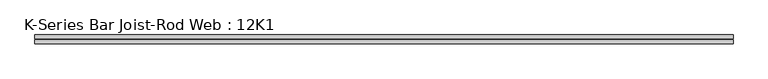
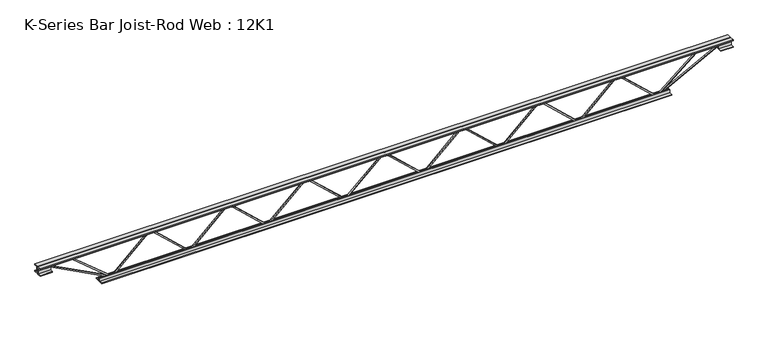
"""IFC4 building model written with IfcOpenShell, lengths in millimetres: beam geometry, K-Series Bar Joist-Rod Web : 12K1."""

import ifcopenshell
import ifcopenshell.guid

model = None  # the IFC model being written
_history = None  # IfcOwnerHistory: only IFC2X3 demands one
_inside = {}  # id of a spatial element -> (the spatial element, [elements in it])
_under = {}  # id of a project, library or spatial element -> (it, [spatial elements below it])
_declared = {}  # id of a project -> (the project, [libraries it declares])
_typed = {}  # id of a type object -> (the type object, [elements of that type])
_made_of = {}  # id of a material, layer set ... -> (it, [elements and type objects made of it])


def new_model(schema):
    """Start an empty IFC model of exactly this schema.

    Asked for "IFC4X3", IfcOpenShell would pick the latest addendum, in which some entities
    have other attributes; the version numbers below select the first issue.
    IFC2X3 requires an IfcOwnerHistory on every rooted entity: one is made here for all.
    """
    global model, _history
    if schema == "IFC4X3":
        model = ifcopenshell.file(schema_version=(4, 3, 0, 0))
    else:
        model = ifcopenshell.file(schema=schema)
    _inside.clear()
    _under.clear()
    _declared.clear()
    _typed.clear()
    _made_of.clear()
    _history = None
    if model.schema == "IFC2X3":
        org = make("IfcOrganization", Name="unknown")
        user = make(
            "IfcPersonAndOrganization",
            ThePerson=make("IfcPerson", FamilyName="unknown"),
            TheOrganization=org,
        )
        app = make(
            "IfcApplication",
            ApplicationDeveloper=org,
            Version="unknown",
            ApplicationFullName="unknown",
            ApplicationIdentifier="unknown",
        )
        _history = make(
            "IfcOwnerHistory",
            OwningUser=user,
            OwningApplication=app,
            ChangeAction="ADDED",
            CreationDate=0,
        )
    return model


def make(cls, **values):
    """One entity of the class cls with the attributes given. An attribute that is None is left unset."""
    return model.create_entity(
        cls, **{name: value for name, value in values.items() if value is not None}
    )


def rooted(cls, **values):
    """An entity with a GlobalId (a new one), such as an element, a storey or a relation."""
    return make(cls, GlobalId=ifcopenshell.guid.new(), OwnerHistory=_history, **values)


def si_unit(unit_type, name, prefix=None):
    """IfcSIUnit, for example si_unit("LENGTHUNIT", "METRE", prefix="MILLI")."""
    return make("IfcSIUnit", UnitType=unit_type, Prefix=prefix, Name=name)


def assignment(units):
    """IfcUnitAssignment: the units of a project."""
    return None if units is None else make("IfcUnitAssignment", Units=units)


def point(xyz):
    """IfcCartesianPoint."""
    return None if xyz is None else make("IfcCartesianPoint", Coordinates=xyz)


def direction(xyz):
    """IfcDirection."""
    return None if xyz is None else make("IfcDirection", DirectionRatios=xyz)


def frame(location, z_axis=None, x_axis=None):
    """IfcAxis2Placement3D, a coordinate frame: its origin and axes. An axis left out is left unset."""
    return make(
        "IfcAxis2Placement3D",
        Location=point(location),
        Axis=direction(z_axis),
        RefDirection=direction(x_axis),
    )


def origin():
    """The frame at (0, 0, 0) with its axes left unset."""
    return frame((0.0, 0.0, 0.0))


def place(relative_to, where):
    """IfcLocalPlacement: puts the frame where relative to a parent placement (None: the world)."""
    return make(
        "IfcLocalPlacement", PlacementRelTo=relative_to, RelativePlacement=where
    )


def context(
    kind, dimensions, precision=None, world=None, true_north=None, identifier=None
):
    """IfcGeometricRepresentationContext, for example the 3D "Model" context."""
    return make(
        "IfcGeometricRepresentationContext",
        ContextIdentifier=identifier,
        ContextType=kind,
        CoordinateSpaceDimension=dimensions,
        Precision=precision,
        WorldCoordinateSystem=world,
        TrueNorth=true_north,
    )


def project(units=None, contexts=None):
    """IfcProject with its units and contexts."""
    return rooted(
        "IfcProject",
        Name="project",
        RepresentationContexts=contexts,
        UnitsInContext=assignment(units),
    )


def spatial(cls, under=None, at=None, **own):
    """A site, building, storey or space (cls), placed at a placement, below another one or the project."""
    s = rooted(cls, ObjectPlacement=at, **own)
    if under is not None:
        _under.setdefault(under.id(), (under, []))[1].append(s)
    return s


def polyline(points):
    """IfcPolyline through the points."""
    return make("IfcPolyline", Points=[point(p) for p in points])


def outline(outer, holes=None, kind="AREA"):
    """IfcArbitraryClosedProfileDef: a profile drawn as a closed curve; with holes, ...WithVoids."""
    if holes is None:
        return make("IfcArbitraryClosedProfileDef", ProfileType=kind, OuterCurve=outer)
    return make(
        "IfcArbitraryProfileDefWithVoids",
        ProfileType=kind,
        OuterCurve=outer,
        InnerCurves=holes,
    )


def extrude(swept, where, along, depth):
    """IfcExtrudedAreaSolid: the profile swept, set in the frame where, extruded along a direction by depth."""
    return make(
        "IfcExtrudedAreaSolid",
        SweptArea=swept,
        Position=where,
        ExtrudedDirection=direction(along),
        Depth=depth,
    )


def shape(context_of_items, identifier, shape_type, items):
    """IfcShapeRepresentation: the items that make up one representation, for example the "Body"."""
    return make(
        "IfcShapeRepresentation",
        ContextOfItems=context_of_items,
        RepresentationIdentifier=identifier,
        RepresentationType=shape_type,
        Items=items,
    )


def source(mapping_origin, context_of_items, identifier, shape_type, items):
    """IfcRepresentationMap: a shape defined once, which mapped items show again and again."""
    return make(
        "IfcRepresentationMap",
        MappingOrigin=mapping_origin,
        MappedRepresentation=shape(context_of_items, identifier, shape_type, items),
    )


def transform(
    local_origin,
    x_axis=None,
    y_axis=None,
    z_axis=None,
    scale=None,
    scale2=None,
    scale3=None,
    uniform=True,
):
    """IfcCartesianTransformationOperator3D, or its non-uniform kind. x_axis, y_axis, z_axis: its Axis1, 2, 3."""
    if uniform:
        return make(
            "IfcCartesianTransformationOperator3D",
            Axis1=direction(x_axis),
            Axis2=direction(y_axis),
            LocalOrigin=point(local_origin),
            Scale=scale,
            Axis3=direction(z_axis),
        )
    return make(
        "IfcCartesianTransformationOperator3DnonUniform",
        Axis1=direction(x_axis),
        Axis2=direction(y_axis),
        LocalOrigin=point(local_origin),
        Scale=scale,
        Axis3=direction(z_axis),
        Scale2=scale2,
        Scale3=scale3,
    )


def mapped(mapping_source, mapping_target):
    """IfcMappedItem: shows the shape of a source again, moved by a transform."""
    return make(
        "IfcMappedItem", MappingSource=mapping_source, MappingTarget=mapping_target
    )


def made_of(thing, what):
    """Note that an element or type object is made of a material, layer set ...; save() writes the relation."""
    if what is not None:
        _made_of.setdefault(what.id(), (what, []))[1].append(thing)
    return thing


def element(
    cls,
    number,
    at=None,
    inside=None,
    cuts=None,
    type_object=None,
    material=None,
    context=None,
    identifier="Body",
    shape_type=None,
    held_by="IfcProductDefinitionShape",
    body=None,
    shapes=None,
    **own,
):
    """One element of the class cls, such as IfcWall. Its Tag is "e" and its number.

    at: its placement. inside: the storey or other place that contains it. cuts: it is an
    opening in that element (IfcRelVoidsElement). A single representation is given by context,
    identifier, shape_type and body (its items); several are given by shapes. held_by: the class
    of the entity that holds the representations. save() writes the other relations.
    """
    e = rooted(cls, Tag="e%d" % number, ObjectPlacement=at, **own)
    if body is not None:
        shapes = [shape(context, identifier, shape_type, body)]
    if shapes is not None:
        e.Representation = make(held_by, Representations=shapes)
    if inside is not None:
        _inside.setdefault(inside.id(), (inside, []))[1].append(e)
    if cuts is not None:
        rooted(
            "IfcRelVoidsElement", RelatingBuildingElement=cuts, RelatedOpeningElement=e
        )
    if type_object is not None:
        _typed.setdefault(type_object.id(), (type_object, []))[1].append(e)
    return made_of(e, material)


def aggregate(whole, parts):
    """IfcRelAggregates: a whole, such as a stair, and the parts it consists of."""
    return rooted("IfcRelAggregates", RelatingObject=whole, RelatedObjects=parts)


def save(model, path):
    """Write the relations noted so far, then the file.

    IfcRelAggregates (storeys below a building ...), IfcRelContainedInSpatialStructure (elements
    in a storey), IfcRelDefinesByType, IfcRelAssociatesMaterial and IfcRelDeclares: one each for
    every whole, place, type object, material and project.
    """
    for whole, parts in _under.values():
        aggregate(whole, parts)
    for where, things in _inside.values():
        rooted(
            "IfcRelContainedInSpatialStructure",
            RelatedElements=things,
            RelatingStructure=where,
        )
    for kind, things in _typed.values():
        rooted("IfcRelDefinesByType", RelatedObjects=things, RelatingType=kind)
    for what, things in _made_of.values():
        rooted("IfcRelAssociatesMaterial", RelatedObjects=things, RelatingMaterial=what)
    for by, libraries in _declared.values():
        rooted("IfcRelDeclares", RelatingContext=by, RelatedDefinitions=libraries)
    model.write(path)


def k_series_bar_joist_rod_web_12k1_a6bee375(model_context):
    return source(origin(), model_context, "Body", "SweptSolid", [
        extrude(outline(polyline([(-141.2875, 964.0660714), (-150.8125, 964.0660714), (-150.8125, 969.1093603), (141.2875, 1284.1147175), (141.2875, 1286.7281397), (-150.8125, 1601.7334968), (-150.8125, 1606.7767857), (-141.2875, 1606.7767857), (-141.2875, 1605.4700746), (150.8125, 1290.4647175), (150.8125, 1280.3781397), (-141.2875, 965.3727825), (-141.2875, 964.0660714)])), frame((0.0, -4.7625, 0.0), z_axis=(0.0, 1.0, 0.0), x_axis=(0.0, 0.0, 1.0)), (0.0, 0.0, 1.0), 9.525),
        extrude(outline(polyline([(-141.2875, 321.3553571), (-150.8125, 321.3553571), (-150.8125, 326.3986461), (141.2875, 641.4040032), (141.2875, 644.0174254), (-150.8125, 959.0227825), (-150.8125, 964.0660714), (-141.2875, 964.0660714), (-141.2875, 962.7593603), (150.8125, 647.7540032), (150.8125, 637.6674254), (-141.2875, 322.6620682), (-141.2875, 321.3553571)])), frame((0.0, -4.7625, 0.0), z_axis=(0.0, 1.0, 0.0), x_axis=(0.0, 0.0, 1.0)), (0.0, 0.0, 1.0), 9.525),
        extrude(outline(polyline([(-141.2875, -321.3553571), (-150.8125, -321.3553571), (-150.8125, -316.3120682), (141.2875, -1.3067111), (141.2875, 1.3067111), (-150.8125, 316.3120682), (-150.8125, 321.3553571), (-141.2875, 321.3553571), (-141.2875, 320.0486461), (150.8125, 5.0432889), (150.8125, -5.0432889), (-141.2875, -320.0486461), (-141.2875, -321.3553571)])), frame((0.0, -4.7625, 0.0), z_axis=(0.0, 1.0, 0.0), x_axis=(0.0, 0.0, 1.0)), (0.0, 0.0, 1.0), 9.525),
        extrude(outline(polyline([(-141.2875, -964.0660714), (-150.8125, -964.0660714), (-150.8125, -959.0227825), (141.2875, -644.0174254), (141.2875, -641.4040032), (-150.8125, -326.3986461), (-150.8125, -321.3553571), (-141.2875, -321.3553571), (-141.2875, -322.6620682), (150.8125, -637.6674254), (150.8125, -647.7540032), (-141.2875, -962.7593603), (-141.2875, -964.0660714)])), frame((0.0, -4.7625, 0.0), z_axis=(0.0, 1.0, 0.0), x_axis=(0.0, 0.0, 1.0)), (0.0, 0.0, 1.0), 9.525),
        extrude(outline(polyline([(-141.2875, -1606.7767857), (-150.8125, -1606.7767857), (-150.8125, -1601.7334968), (141.2875, -1286.7281397), (141.2875, -1284.1147175), (-150.8125, -969.1093603), (-150.8125, -964.0660714), (-141.2875, -964.0660714), (-141.2875, -965.3727825), (150.8125, -1280.3781397), (150.8125, -1290.4647175), (-141.2875, -1605.4700746), (-141.2875, -1606.7767857)])), frame((0.0, -4.7625, 0.0), z_axis=(0.0, 1.0, 0.0), x_axis=(0.0, 0.0, 1.0)), (0.0, 0.0, 1.0), 9.525),
        extrude(outline(polyline([(-141.2875, 1606.7767857), (-150.8125, 1606.7767857), (-150.8125, 1611.8200746), (141.2875, 1926.8254318), (141.2875, 1929.4388539), (-150.8125, 2244.4442111), (-150.8125, 2249.4875), (-141.2875, 2249.4875), (-141.2875, 2248.1807889), (150.8125, 1933.1754318), (150.8125, 1923.0888539), (-141.2875, 1608.0834968), (-141.2875, 1606.7767857)])), frame((0.0, -4.7625, 0.0), z_axis=(0.0, 1.0, 0.0), x_axis=(0.0, 0.0, 1.0)), (0.0, 0.0, 1.0), 9.525),
        extrude(outline(polyline([(-141.2875, -2249.4875), (-150.8125, -2249.4875), (-150.8125, -2244.4442111), (141.2875, -1929.4388539), (141.2875, -1926.8254318), (-150.8125, -1611.8200746), (-150.8125, -1606.7767857), (-141.2875, -1606.7767857), (-141.2875, -1608.0834968), (150.8125, -1923.0888539), (150.8125, -1933.1754318), (-141.2875, -2248.1807889), (-141.2875, -2249.4875)])), frame((0.0, -4.7625, 0.0), z_axis=(0.0, 1.0, 0.0), x_axis=(0.0, 0.0, 1.0)), (0.0, 0.0, 1.0), 9.525),
        extrude(outline(polyline([(4.7625, 152.4), (36.5125, 152.4), (36.5125, 146.05), (11.1125, 146.05), (11.1125, 120.65), (4.7625, 120.65), (4.7625, 152.4)])), frame((-2859.0875, 0.0, 0.0), z_axis=(1.0, 0.0, 0.0), x_axis=(0.0, 1.0, 0.0)), (0.0, 0.0, 1.0), 5718.175),
        extrude(outline(polyline([(-4.7625, 152.4), (-4.7625, 120.65), (-11.1125, 120.65), (-11.1125, 146.05), (-36.5125, 146.05), (-36.5125, 152.4), (-4.7625, 152.4)])), frame((-2859.0875, 0.0, 0.0), z_axis=(1.0, 0.0, 0.0), x_axis=(0.0, 1.0, 0.0)), (0.0, 0.0, 1.0), 5718.175),
        extrude(outline(polyline([(-4.7625, 88.9), (-36.5125, 88.9), (-36.5125, 95.25), (-11.1125, 95.25), (-11.1125, 120.65), (-4.7625, 120.65), (-4.7625, 88.9)])), frame((-2859.0875, 0.0, 0.0), z_axis=(1.0, 0.0, 0.0), x_axis=(0.0, 1.0, 0.0)), (0.0, 0.0, 1.0), 101.6),
        extrude(outline(polyline([(36.5125, 88.9), (4.7625, 88.9), (4.7625, 120.65), (11.1125, 120.65), (11.1125, 95.25), (36.5125, 95.25), (36.5125, 88.9)])), frame((-2859.0875, 0.0, 0.0), z_axis=(1.0, 0.0, 0.0), x_axis=(0.0, 1.0, 0.0)), (0.0, 0.0, 1.0), 101.6),
        extrude(outline(polyline([(4.7625, 88.9), (4.7625, 120.65), (11.1125, 120.65), (11.1125, 95.25), (36.5125, 95.25), (36.5125, 88.9), (4.7625, 88.9)])), frame((2757.4875, 0.0, 0.0), z_axis=(1.0, 0.0, 0.0), x_axis=(0.0, 1.0, 0.0)), (0.0, 0.0, 1.0), 101.6),
        extrude(outline(polyline([(-4.7625, 88.9), (-36.5125, 88.9), (-36.5125, 95.25), (-11.1125, 95.25), (-11.1125, 120.65), (-4.7625, 120.65), (-4.7625, 88.9)])), frame((2757.4875, 0.0, 0.0), z_axis=(1.0, 0.0, 0.0), x_axis=(0.0, 1.0, 0.0)), (0.0, 0.0, 1.0), 101.6),
        extrude(outline(polyline([(4.7625, -152.4), (4.7625, -120.65), (11.1125, -120.65), (11.1125, -146.05), (36.5125, -146.05), (36.5125, -152.4), (4.7625, -152.4)])), frame((-2351.0875, 0.0, 0.0), z_axis=(1.0, 0.0, 0.0), x_axis=(0.0, 1.0, 0.0)), (0.0, 0.0, 1.0), 4702.175),
        extrude(outline(polyline([(-4.7625, -152.4), (-36.5125, -152.4), (-36.5125, -146.05), (-11.1125, -146.05), (-11.1125, -120.65), (-4.7625, -120.65), (-4.7625, -152.4)])), frame((-2351.0875, 0.0, 0.0), z_axis=(1.0, 0.0, 0.0), x_axis=(0.0, 1.0, 0.0)), (0.0, 0.0, 1.0), 4702.175),
        extrude(outline(polyline([(0.0, -9.525), (0.0, 0.0), (573.7533355, 0.0), (573.7533355, -9.525), (0.0, -9.525)])), frame((-2759.7012714, 4.7625, 116.4332925), z_axis=(0.46483389898951455, 0.0, 0.8853979028381567), x_axis=(0.8853979028381567, 0.0, -0.46483389898951455)), (0.0, 0.0, 1.0), 9.525),
        extrude(outline(polyline([(0.0, -9.525), (0.0, 0.0), (417.610052, 0.0), (417.610052, -9.525), (0.0, -9.525)])), frame((-2573.8843518, 4.7625, 116.9852058), z_axis=(0.6386340527421636, 0.0, 0.7695105890617228), x_axis=(0.7695105890617228, 0.0, -0.6386340527421636)), (0.0, 0.0, 1.0), 9.525),
        extrude(outline(polyline([(0.0, -9.525), (0.0, 0.0), (573.7533355, 0.0), (573.7533355, -9.525), (0.0, -9.525)])), frame((2759.7012714, -4.7625, 116.4332925), z_axis=(-0.4648338989894956, 0.0, 0.8853979028381666), x_axis=(-0.8853979028381666, 0.0, -0.4648338989894956)), (0.0, 0.0, 1.0), 9.525),
        extrude(outline(polyline([(0.0, -9.525), (0.0, 0.0), (417.610052, 0.0), (417.610052, -9.525), (0.0, -9.525)])), frame((2573.8843518, -4.7625, 116.9852058), z_axis=(-0.6386340527421579, 0.0, 0.7695105890617275), x_axis=(-0.7695105890617275, 0.0, -0.6386340527421579)), (0.0, 0.0, 1.0), 9.525),
    ])


if __name__ == "__main__":
    model = new_model("IFC4")
    model_context = context("Model", 3, world=origin())
    ifc_project = project(units=[si_unit("LENGTHUNIT", "METRE", prefix="MILLI")], contexts=[model_context])
    site = spatial("IfcSite", under=ifc_project)
    building = spatial("IfcBuilding", under=site)
    placement = place(None, origin())
    k_series_bar_joist_rod_web_12k1_shape = k_series_bar_joist_rod_web_12k1_a6bee375(model_context)
    element("IfcBeam", 1, ObjectType="K-Series Bar Joist-Rod Web : 12K1", at=placement, inside=building, context=model_context, shape_type="MappedRepresentation", body=[
        mapped(k_series_bar_joist_rod_web_12k1_shape, transform((0.0, 0.0, 0.0), x_axis=(1.0, 0.0, 0.0), y_axis=(0.0, 1.0, 0.0), z_axis=(0.0, 0.0, 1.0))),
    ])
    save(model, "model.ifc")

# Revit data of these elements
# Type "K-Series Bar Joist-Rod Web : 12K1"
#   Assembly Code = "B1010350"
#   Wt = 5
#   Web Thickness = 9.525 mm
#   Start Offset [instance default] = 0 mm
#   Start Extension [instance default] = 0 mm
#   Seat Length = 101.6 mm
#   Seat Depth = 63.5 mm
#   PanelArrayLength [instance default] = 6096 mm
#   Panel [instance default] = 609.6 mm
#   End Offset [instance default] = 0 mm
#   End Extension [instance default] = 0 mm
#   End Panel = 609.6 mm
#   Cord Leg = 31.75 mm
#   Chord Thickness = 6.35 mm
#   Length [instance default] = 7315.2 mm
#   Depth = 304.8 mm
#   PanelArrayNum [instance default] = 10
#   Structural Material = Steel ASTM A500, Grade C, Round
# Element 1 (IfcBeam, "K-Series Bar Joist-Rod Web : 12K1")
#   PanelArrayLength = 4498.975 mm
#   Panel = 642.711 mm
#   PanelArrayNum = 7
#   Materials on its faces: "Steel ASTM A500, Grade C, Round"
# Materials
#   "Steel ASTM A500, Grade C, Round": class "Metal", colour RGB 202 101 0, transparency 0, Description = "Carbon steel", Cost = 0
